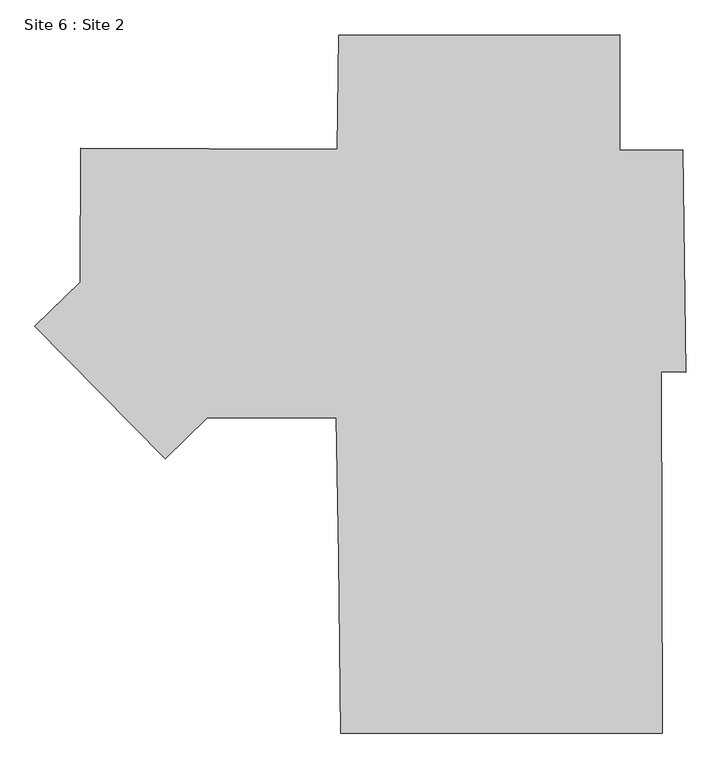
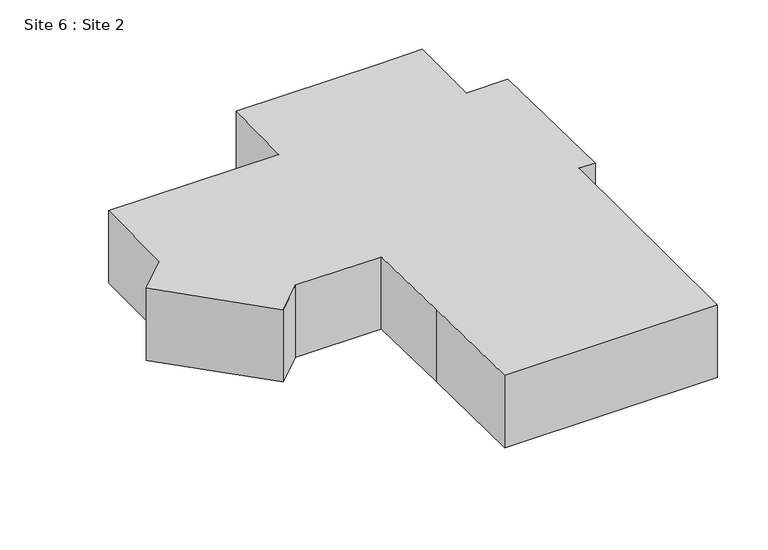
"""IFC4 building model written with IfcOpenShell, lengths in millimetres: geographic element geometry, Site 6 : Site 2."""

import ifcopenshell
import ifcopenshell.guid

model = None  # the IFC model being written
_history = None  # IfcOwnerHistory: only IFC2X3 demands one
_inside = {}  # id of a spatial element -> (the spatial element, [elements in it])
_under = {}  # id of a project, library or spatial element -> (it, [spatial elements below it])
_declared = {}  # id of a project -> (the project, [libraries it declares])
_typed = {}  # id of a type object -> (the type object, [elements of that type])
_made_of = {}  # id of a material, layer set ... -> (it, [elements and type objects made of it])


def new_model(schema):
    """Start an empty IFC model of exactly this schema.

    Asked for "IFC4X3", IfcOpenShell would pick the latest addendum, in which some entities
    have other attributes; the version numbers below select the first issue.
    IFC2X3 requires an IfcOwnerHistory on every rooted entity: one is made here for all.
    """
    global model, _history
    if schema == "IFC4X3":
        model = ifcopenshell.file(schema_version=(4, 3, 0, 0))
    else:
        model = ifcopenshell.file(schema=schema)
    _inside.clear()
    _under.clear()
    _declared.clear()
    _typed.clear()
    _made_of.clear()
    _history = None
    if model.schema == "IFC2X3":
        org = make("IfcOrganization", Name="unknown")
        user = make(
            "IfcPersonAndOrganization",
            ThePerson=make("IfcPerson", FamilyName="unknown"),
            TheOrganization=org,
        )
        app = make(
            "IfcApplication",
            ApplicationDeveloper=org,
            Version="unknown",
            ApplicationFullName="unknown",
            ApplicationIdentifier="unknown",
        )
        _history = make(
            "IfcOwnerHistory",
            OwningUser=user,
            OwningApplication=app,
            ChangeAction="ADDED",
            CreationDate=0,
        )
    return model


def make(cls, **values):
    """One entity of the class cls with the attributes given. An attribute that is None is left unset."""
    return model.create_entity(
        cls, **{name: value for name, value in values.items() if value is not None}
    )


def rooted(cls, **values):
    """An entity with a GlobalId (a new one), such as an element, a storey or a relation."""
    return make(cls, GlobalId=ifcopenshell.guid.new(), OwnerHistory=_history, **values)


def si_unit(unit_type, name, prefix=None):
    """IfcSIUnit, for example si_unit("LENGTHUNIT", "METRE", prefix="MILLI")."""
    return make("IfcSIUnit", UnitType=unit_type, Prefix=prefix, Name=name)


def assignment(units):
    """IfcUnitAssignment: the units of a project."""
    return None if units is None else make("IfcUnitAssignment", Units=units)


def point(xyz):
    """IfcCartesianPoint."""
    return None if xyz is None else make("IfcCartesianPoint", Coordinates=xyz)


def direction(xyz):
    """IfcDirection."""
    return None if xyz is None else make("IfcDirection", DirectionRatios=xyz)


def frame(location, z_axis=None, x_axis=None):
    """IfcAxis2Placement3D, a coordinate frame: its origin and axes. An axis left out is left unset."""
    return make(
        "IfcAxis2Placement3D",
        Location=point(location),
        Axis=direction(z_axis),
        RefDirection=direction(x_axis),
    )


def origin():
    """The frame at (0, 0, 0) with its axes left unset."""
    return frame((0.0, 0.0, 0.0))


def place(relative_to, where):
    """IfcLocalPlacement: puts the frame where relative to a parent placement (None: the world)."""
    return make(
        "IfcLocalPlacement", PlacementRelTo=relative_to, RelativePlacement=where
    )


def context(
    kind, dimensions, precision=None, world=None, true_north=None, identifier=None
):
    """IfcGeometricRepresentationContext, for example the 3D "Model" context."""
    return make(
        "IfcGeometricRepresentationContext",
        ContextIdentifier=identifier,
        ContextType=kind,
        CoordinateSpaceDimension=dimensions,
        Precision=precision,
        WorldCoordinateSystem=world,
        TrueNorth=true_north,
    )


def project(units=None, contexts=None):
    """IfcProject with its units and contexts."""
    return rooted(
        "IfcProject",
        Name="project",
        RepresentationContexts=contexts,
        UnitsInContext=assignment(units),
    )


def spatial(cls, under=None, at=None, **own):
    """A site, building, storey or space (cls), placed at a placement, below another one or the project."""
    s = rooted(cls, ObjectPlacement=at, **own)
    if under is not None:
        _under.setdefault(under.id(), (under, []))[1].append(s)
    return s


def polyline(points):
    """IfcPolyline through the points."""
    return make("IfcPolyline", Points=[point(p) for p in points])


def outline(outer, holes=None, kind="AREA"):
    """IfcArbitraryClosedProfileDef: a profile drawn as a closed curve; with holes, ...WithVoids."""
    if holes is None:
        return make("IfcArbitraryClosedProfileDef", ProfileType=kind, OuterCurve=outer)
    return make(
        "IfcArbitraryProfileDefWithVoids",
        ProfileType=kind,
        OuterCurve=outer,
        InnerCurves=holes,
    )


def extrude(swept, where, along, depth):
    """IfcExtrudedAreaSolid: the profile swept, set in the frame where, extruded along a direction by depth."""
    return make(
        "IfcExtrudedAreaSolid",
        SweptArea=swept,
        Position=where,
        ExtrudedDirection=direction(along),
        Depth=depth,
    )


def shape(context_of_items, identifier, shape_type, items):
    """IfcShapeRepresentation: the items that make up one representation, for example the "Body"."""
    return make(
        "IfcShapeRepresentation",
        ContextOfItems=context_of_items,
        RepresentationIdentifier=identifier,
        RepresentationType=shape_type,
        Items=items,
    )


def source(mapping_origin, context_of_items, identifier, shape_type, items):
    """IfcRepresentationMap: a shape defined once, which mapped items show again and again."""
    return make(
        "IfcRepresentationMap",
        MappingOrigin=mapping_origin,
        MappedRepresentation=shape(context_of_items, identifier, shape_type, items),
    )


def transform(
    local_origin,
    x_axis=None,
    y_axis=None,
    z_axis=None,
    scale=None,
    scale2=None,
    scale3=None,
    uniform=True,
):
    """IfcCartesianTransformationOperator3D, or its non-uniform kind. x_axis, y_axis, z_axis: its Axis1, 2, 3."""
    if uniform:
        return make(
            "IfcCartesianTransformationOperator3D",
            Axis1=direction(x_axis),
            Axis2=direction(y_axis),
            LocalOrigin=point(local_origin),
            Scale=scale,
            Axis3=direction(z_axis),
        )
    return make(
        "IfcCartesianTransformationOperator3DnonUniform",
        Axis1=direction(x_axis),
        Axis2=direction(y_axis),
        LocalOrigin=point(local_origin),
        Scale=scale,
        Axis3=direction(z_axis),
        Scale2=scale2,
        Scale3=scale3,
    )


def mapped(mapping_source, mapping_target):
    """IfcMappedItem: shows the shape of a source again, moved by a transform."""
    return make(
        "IfcMappedItem", MappingSource=mapping_source, MappingTarget=mapping_target
    )


def made_of(thing, what):
    """Note that an element or type object is made of a material, layer set ...; save() writes the relation."""
    if what is not None:
        _made_of.setdefault(what.id(), (what, []))[1].append(thing)
    return thing


def element(
    cls,
    number,
    at=None,
    inside=None,
    cuts=None,
    type_object=None,
    material=None,
    context=None,
    identifier="Body",
    shape_type=None,
    held_by="IfcProductDefinitionShape",
    body=None,
    shapes=None,
    **own,
):
    """One element of the class cls, such as IfcWall. Its Tag is "e" and its number.

    at: its placement. inside: the storey or other place that contains it. cuts: it is an
    opening in that element (IfcRelVoidsElement). A single representation is given by context,
    identifier, shape_type and body (its items); several are given by shapes. held_by: the class
    of the entity that holds the representations. save() writes the other relations.
    """
    e = rooted(cls, Tag="e%d" % number, ObjectPlacement=at, **own)
    if body is not None:
        shapes = [shape(context, identifier, shape_type, body)]
    if shapes is not None:
        e.Representation = make(held_by, Representations=shapes)
    if inside is not None:
        _inside.setdefault(inside.id(), (inside, []))[1].append(e)
    if cuts is not None:
        rooted(
            "IfcRelVoidsElement", RelatingBuildingElement=cuts, RelatedOpeningElement=e
        )
    if type_object is not None:
        _typed.setdefault(type_object.id(), (type_object, []))[1].append(e)
    return made_of(e, material)


def aggregate(whole, parts):
    """IfcRelAggregates: a whole, such as a stair, and the parts it consists of."""
    return rooted("IfcRelAggregates", RelatingObject=whole, RelatedObjects=parts)


def save(model, path):
    """Write the relations noted so far, then the file.

    IfcRelAggregates (storeys below a building ...), IfcRelContainedInSpatialStructure (elements
    in a storey), IfcRelDefinesByType, IfcRelAssociatesMaterial and IfcRelDeclares: one each for
    every whole, place, type object, material and project.
    """
    for whole, parts in _under.values():
        aggregate(whole, parts)
    for where, things in _inside.values():
        rooted(
            "IfcRelContainedInSpatialStructure",
            RelatedElements=things,
            RelatingStructure=where,
        )
    for kind, things in _typed.values():
        rooted("IfcRelDefinesByType", RelatedObjects=things, RelatingType=kind)
    for what, things in _made_of.values():
        rooted("IfcRelAssociatesMaterial", RelatedObjects=things, RelatingMaterial=what)
    for by, libraries in _declared.values():
        rooted("IfcRelDeclares", RelatingContext=by, RelatedDefinitions=libraries)
    model.write(path)


def site_6_site_2_d98898f6(model_context):
    return source(origin(), model_context, "Body", "SweptSolid", [
        extrude(outline(polyline([(-15214.7871008, 111231.0905537), (-11048.1543414, 111272.3359659), (-10855.197666, 96536.2310929), (-12480.6255393, 96559.7790667), (-12420.1240701, 72680.7905545), (-33656.7098652, 72683.6248607), (-33793.7026636, 84269.05712), (-33964.5413496, 93517.9430993), (-42499.5178675, 93539.9829585), (-45282.1665111, 90836.8254736), (-53893.7525646, 99598.386294), (-50904.9826146, 102501.7322056), (-50878.53392, 111341.3262468), (-33910.1680098, 111298.718246), (-33801.2602868, 118816.2078743), (-19575.8102621, 118813.3371712), (-15205.9990186, 118851.6390867), (-15214.7871008, 111231.0905537)])), frame((0.0, 0.0, 266395.2), z_axis=(0.0, 0.0, 1.0), x_axis=(1.0, 0.0, 0.0)), (0.0, 0.0, 1.0), 7620.0),
    ])


if __name__ == "__main__":
    model = new_model("IFC4")
    model_context = context("Model", 3, world=origin())
    ifc_project = project(units=[si_unit("LENGTHUNIT", "METRE", prefix="MILLI")], contexts=[model_context])
    site = spatial("IfcSite", under=ifc_project)
    building = spatial("IfcBuilding", under=site)
    placement = place(None, origin())
    site_6_site_2_shape = site_6_site_2_d98898f6(model_context)
    element("IfcGeographicElement", 1, ObjectType="Site 6 : Site 2", at=placement, inside=building, context=model_context, shape_type="MappedRepresentation", body=[
        mapped(site_6_site_2_shape, transform((0.0, 0.0, 0.0), x_axis=(1.0, 0.0, 0.0), y_axis=(0.0, 1.0, 0.0), z_axis=(0.0, 0.0, 1.0))),
    ])
    save(model, "model.ifc")

# Revit data of these elements
# Element 1 (IfcGeographicElement, "Site 6 : Site 2")
#   Materials on its faces: "EXISTING BUILDING"
# Materials
#   "EXISTING BUILDING": class "Generic", colour RGB 120 120 120, transparency 0, Cost = 0
